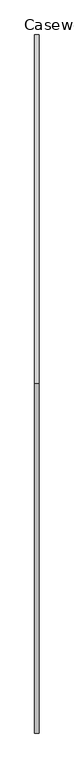
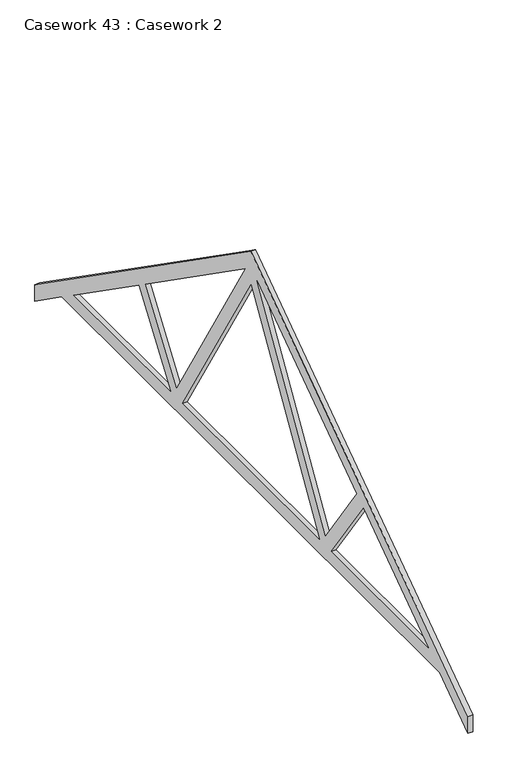
"""IFC4 building model written with IfcOpenShell, lengths in millimetres: furniture geometry, Casework 43 : Casework 2."""

from ifc_helpers import new_model, si_unit, frame, origin, place, context, project, spatial, polyline, outline, extrude, source, transform, mapped, element, save


def casework_43_casework_2_e74e5d3e(model_context):
    return source(origin(), model_context, "Body", "SweptSolid", [
        extrude(outline(polyline([(6583.1149316, 5257.5), (-277.3850684, 5257.5), (-786.6126654, 4900.9349979), (-786.6126654, 5084.0511862), (3152.8649316, 7842.5030963), (7073.1149316, 5097.5144946), (7073.1149316, 4914.3983063), (6583.1149316, 5257.5)]), holes=[polyline([(4612.3149663, 5407.5), (6368.8927306, 5407.5), (5190.2113591, 6232.8215815), (4612.3149663, 5407.5)]), polyline([(4394.2037684, 5407.5), (3152.8649316, 7473.4347567), (1911.5260948, 5407.5), (4394.2037684, 5407.5)]), polyline([(4504.5438357, 5515.1038939), (5067.3385525, 6318.8580469), (3262.0771677, 7582.915677), (4504.5438357, 5515.1038939)]), polyline([(1693.4148969, 5407.5), (1115.5185041, 6232.8215815), (-63.1628674, 5407.5), (1693.4148969, 5407.5)]), polyline([(1801.1860276, 5515.1038939), (3043.6526956, 7582.915677), (1238.3913108, 6318.8580469), (1801.1860276, 5515.1038939)])]), frame((-8621.5247381, 0.0, 0.0), z_axis=(1.0, 0.0, 0.0), x_axis=(0.0, 1.0, 0.0)), (0.0, 0.0, 1.0), 49.6351915),
    ])


if __name__ == "__main__":
    model = new_model("IFC4")
    model_context = context("Model", 3, world=origin())
    ifc_project = project(units=[si_unit("LENGTHUNIT", "METRE", prefix="MILLI")], contexts=[model_context])
    site = spatial("IfcSite", under=ifc_project)
    building = spatial("IfcBuilding", under=site)
    placement = place(None, origin())
    casework_43_casework_2_shape = casework_43_casework_2_e74e5d3e(model_context)
    element("IfcFurniture", 1, ObjectType="Casework 43 : Casework 2", at=placement, inside=building, context=model_context, shape_type="MappedRepresentation", body=[
        mapped(casework_43_casework_2_shape, transform((0.0, 0.0, 0.0), x_axis=(1.0, 0.0, 0.0), y_axis=(0.0, 1.0, 0.0), z_axis=(0.0, 0.0, 1.0))),
    ])
    save(model, "model.ifc")

# Revit data of these elements
# Element 1 (IfcFurniture, "Casework 43 : Casework 2")
#   Materials on its faces: "Softwood, Lumber"
# Materials
#   "Softwood, Lumber": class "Wood", colour RGB 205 156 65, transparency 0, Description = "Pinus Echinata", Cost = 0
